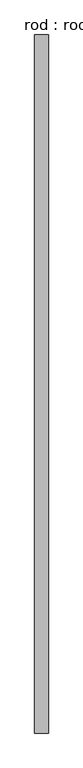
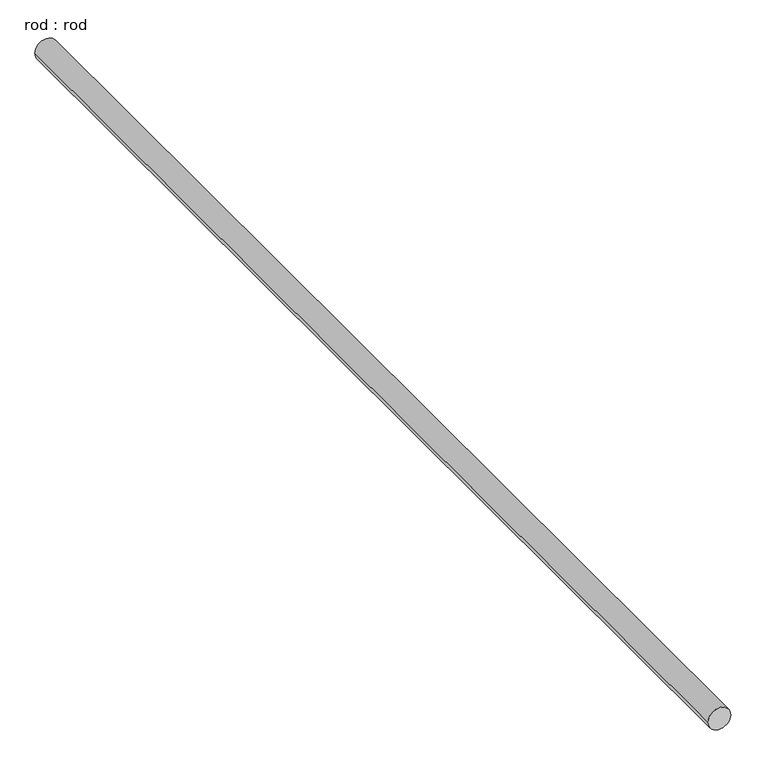
"""IFC4 building model written with IfcOpenShell, lengths in millimetres: proxy geometry, rod : rod."""

from ifc_helpers import new_model, si_unit, point, frame, frame_2d, origin, place, context, project, spatial, circle_curve, trimmed, segment, composite_curve, outline, extrude, source, transform, mapped, element, save


def rod_rod_5b1264ed(model_context):
    return source(origin(), model_context, "Body", "SweptSolid", [
        extrude(outline(composite_curve([segment(trimmed(circle_curve(frame_2d((0.0108462, 0.0)), 200.0), [point((0.0108462, 200.0))], [point((0.0108462, -200.0))], False, "CARTESIAN"), True, "CONTINUOUS"), segment(trimmed(circle_curve(frame_2d((0.0108462, 0.0)), 200.0), [point((0.0108462, -200.0))], [point((0.0108462, 200.0))], False, "CARTESIAN"), True, "CONTINUOUS")], self_intersect=False)), frame((0.0, -6157.2713847, 0.0), z_axis=(0.0, 1.0, 0.0), x_axis=(0.0, 0.0, 1.0)), (0.0, 0.0, 1.0), 20500.0),
    ])


if __name__ == "__main__":
    model = new_model("IFC4")
    model_context = context("Model", 3, world=origin())
    ifc_project = project(units=[si_unit("LENGTHUNIT", "METRE", prefix="MILLI")], contexts=[model_context])
    site = spatial("IfcSite", under=ifc_project)
    building = spatial("IfcBuilding", under=site)
    placement = place(None, origin())
    rod_rod_shape = rod_rod_5b1264ed(model_context)
    element("IfcBuildingElementProxy", 1, Name="rod : rod", ObjectType="rod : rod", at=placement, inside=building, context=model_context, shape_type="MappedRepresentation", body=[
        mapped(rod_rod_shape, transform((0.0, 0.0, 0.0), x_axis=(1.0, 0.0, 0.0), y_axis=(0.0, 1.0, 0.0), z_axis=(0.0, 0.0, 1.0))),
    ])
    save(model, "model.ifc")

# Revit data of these elements
# Type "rod : rod"
#   Default Elevation = 0
